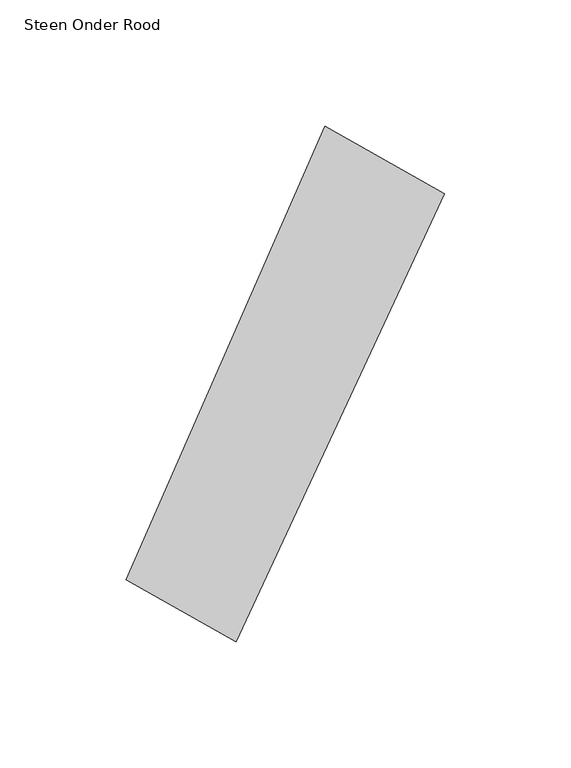
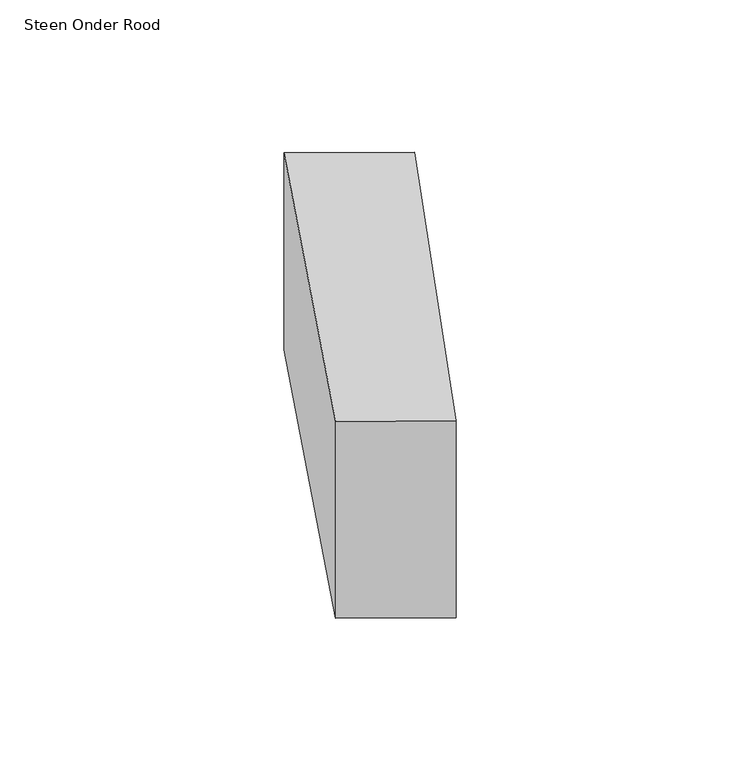
"""IFC4 building model written with IfcOpenShell, lengths in millimetres: proxy geometry, 00_GMA_steen_versie_4 : Steen Onder Rood."""

from ifc_helpers import new_model, si_unit, origin, origin_with_axes, place, context, project, spatial, polyline, outline, extrude, source, transform, mapped, element, save


def steen_onder_rood_1153672e(model_context):
    return source(origin(), model_context, "Body", "SweptSolid", [
        extrude(outline(polyline([(141.4126251, 157.4535719), (58.8725706, -19.8833116), (15.3147161, 4.6669087), (94.0826617, 184.1393015), (141.4126251, 157.4535719)])), origin_with_axes(), (0.0, 0.0, 1.0), 100.0),
    ])


if __name__ == "__main__":
    model = new_model("IFC4")
    model_context = context("Model", 3, world=origin())
    ifc_project = project(units=[si_unit("LENGTHUNIT", "METRE", prefix="MILLI")], contexts=[model_context])
    site = spatial("IfcSite", under=ifc_project)
    building = spatial("IfcBuilding", under=site)
    placement = place(None, origin())
    steen_onder_rood_shape = steen_onder_rood_1153672e(model_context)
    element("IfcBuildingElementProxy", 1, Name="00_GMA_steen_versie_4 : Steen Onder Rood", ObjectType="00_GMA_steen_versie_4 : Steen Onder Rood", at=placement, inside=building, context=model_context, shape_type="MappedRepresentation", body=[
        mapped(steen_onder_rood_shape, transform((0.0, 0.0, 0.0), x_axis=(1.0, 0.0, 0.0), y_axis=(0.0, 1.0, 0.0), z_axis=(0.0, 0.0, 1.0))),
    ])
    save(model, "model.ifc")

# Revit data of these elements
# Type "00_GMA_steen_versie_4 : Steen Onder Rood"
#   StootVoegHalfBoven [instance default] = 5 mm
#   StootVoegHalf [instance default] = 5 mm
#   StootVoegBreedteOnder = 10 mm
#   StootVoegBreedteBoven = 10 mm
#   Steendikte = 100 mm
#   LintVoegOnderHalf = 0 mm
#   LintVoegOnder = 0 mm
#   LintVoegBovenHalf = 5 mm
#   LintVoegBoven = 10 mm
#   materiaal = 21_steen_rood
#   MateriaalVoeg = none
#   Default Elevation = 0
# Element 1 (IfcBuildingElementProxy, "00_GMA_steen_versie_4 : Steen Onder Rood")
#   Materials on its faces: "21_steen_rood"
# Materials
#   "21_steen_rood": class "Unassigned", colour RGB 213 111 43, transparency 0, Cost = 0
